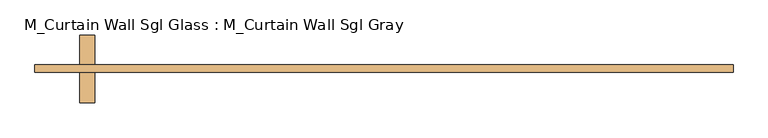
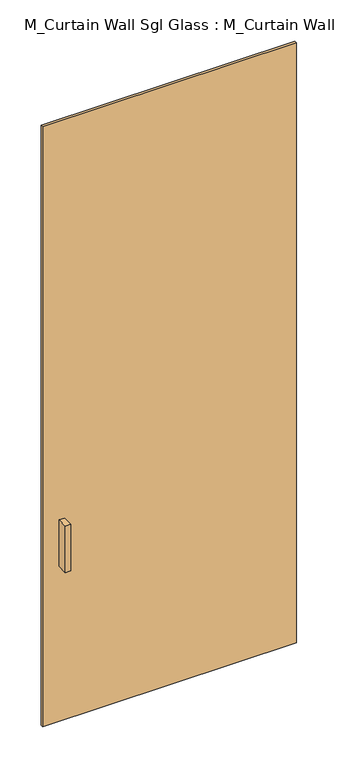
"""IFC4 building model written with IfcOpenShell, lengths in millimetres: door geometry, M_Curtain Wall Sgl Glass : M_Curtain Wall Sgl Gray."""

from ifc_helpers import new_model, si_unit, frame, origin, origin_with_axes, place, context, project, spatial, polyline, outline, extrude, source, transform, mapped, element, save


def m_curtain_wall_sgl_glass_m_curtain_wall_sgl_gray_1afa9b59(model_context):
    return source(origin(), model_context, "Body", "SweptSolid", [
        extrude(outline(polyline([(-489.4881009, -12.5), (-514.8881009, -12.5), (-514.8881009, 38.3), (-489.4881009, 38.3), (-489.4881009, -12.5)])), frame((0.0, 0.0, 762.0), z_axis=(0.0, 0.0, 1.0), x_axis=(1.0, 0.0, 0.0)), (0.0, 0.0, 1.0), 228.6),
        extrude(outline(polyline([(-514.8881009, 101.8), (-489.4881009, 101.8), (-489.4881009, 51.0), (-514.8881009, 51.0), (-514.8881009, 101.8)])), frame((0.0, 0.0, 762.0), z_axis=(0.0, 0.0, 1.0), x_axis=(1.0, 0.0, 0.0)), (0.0, 0.0, 1.0), 228.6),
        extrude(outline(polyline([(591.0881009, 51.0), (591.0881009, 38.3), (-591.0881009, 38.3), (-591.0881009, 51.0), (591.0881009, 51.0)])), origin_with_axes(), (0.0, 0.0, 1.0), 2950.0),
    ])


if __name__ == "__main__":
    model = new_model("IFC4")
    model_context = context("Model", 3, world=origin())
    ifc_project = project(units=[si_unit("LENGTHUNIT", "METRE", prefix="MILLI")], contexts=[model_context])
    site = spatial("IfcSite", under=ifc_project)
    building = spatial("IfcBuilding", under=site)
    placement = place(None, origin())
    m_curtain_wall_sgl_glass_m_curtain_wall_sgl_gray_shape = m_curtain_wall_sgl_glass_m_curtain_wall_sgl_gray_1afa9b59(model_context)
    element("IfcDoor", 1, ObjectType="M_Curtain Wall Sgl Glass : M_Curtain Wall Sgl Gray", at=placement, inside=building, context=model_context, shape_type="MappedRepresentation", body=[
        mapped(m_curtain_wall_sgl_glass_m_curtain_wall_sgl_gray_shape, transform((0.0, 0.0, 0.0), x_axis=(1.0, 0.0, 0.0), y_axis=(0.0, 1.0, 0.0), z_axis=(0.0, 0.0, 1.0))),
    ])
    save(model, "model.ifc")

# Revit data of these elements
# Type "M_Curtain Wall Sgl Glass : M_Curtain Wall Sgl Gray"
#   Model = "12345667"
#   Manufacturer = "Dublin Doors"
#   Description = "Single Flush door"
#   Type Mark = "48"
#   COBie.Type.CreatedBy = "design@eagle.com"
#   COBie.Type.CreatedOn = "2016-09-13T05:47:35"
#   COBie.Type.Name = "Doors_M_Curtain Wall Sgl Glass_M_Curtain Wall Sgl Gray"
#   COBie.Type.Category = "23-30 10 00 : Doors"
#   COBie.Type.Description = "Single Flush door"
#   COBie.Type.Manufacturer = "Dublin Doors"
#   COBie.Type.ModelNumber = "12345667"
#   Construction Type Id = "opn-d36"
#   Analytic Construction = "Wood panel"
#   COBie.Type.ReplacementCost = 0
#   Offset = 51 mm
#   Heat Transfer Coefficient (U) = 3.8042 W/(m²·K)
#   COBie.Type = yes
#   Function = 1
#   Glazing Material = Door - Frame(1)
#   Visual Light Transmittance = 0
#   Solar Heat Gain Coefficient = 0
# Element 1 (IfcDoor, "M_Curtain Wall Sgl Glass : M_Curtain Wall Sgl Gray")
#   Materials on its faces: "Aluminum", "Door - Frame(1)"
# Materials
#   "Door - Frame(1)": class "Miscellaneous", colour RGB 128 128 128, transparency 0, Cost = 0
#   "Aluminum": class "Metal", colour RGB 247 247 247, transparency 0, Description = "Aluminum 6061", Cost = 0
